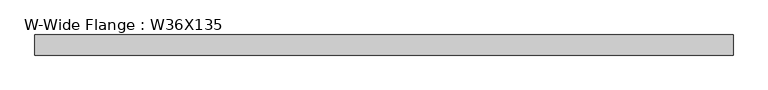
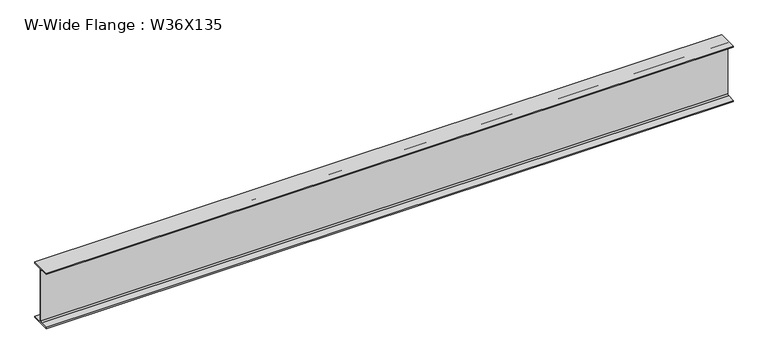
"""IFC4 building model written with IfcOpenShell, lengths in millimetres: beam geometry, W-Wide Flange : W36X135."""

import ifcopenshell
import ifcopenshell.guid

model = None  # the IFC model being written
_history = None  # IfcOwnerHistory: only IFC2X3 demands one
_inside = {}  # id of a spatial element -> (the spatial element, [elements in it])
_under = {}  # id of a project, library or spatial element -> (it, [spatial elements below it])
_declared = {}  # id of a project -> (the project, [libraries it declares])
_typed = {}  # id of a type object -> (the type object, [elements of that type])
_made_of = {}  # id of a material, layer set ... -> (it, [elements and type objects made of it])


def new_model(schema):
    """Start an empty IFC model of exactly this schema.

    Asked for "IFC4X3", IfcOpenShell would pick the latest addendum, in which some entities
    have other attributes; the version numbers below select the first issue.
    IFC2X3 requires an IfcOwnerHistory on every rooted entity: one is made here for all.
    """
    global model, _history
    if schema == "IFC4X3":
        model = ifcopenshell.file(schema_version=(4, 3, 0, 0))
    else:
        model = ifcopenshell.file(schema=schema)
    _inside.clear()
    _under.clear()
    _declared.clear()
    _typed.clear()
    _made_of.clear()
    _history = None
    if model.schema == "IFC2X3":
        org = make("IfcOrganization", Name="unknown")
        user = make(
            "IfcPersonAndOrganization",
            ThePerson=make("IfcPerson", FamilyName="unknown"),
            TheOrganization=org,
        )
        app = make(
            "IfcApplication",
            ApplicationDeveloper=org,
            Version="unknown",
            ApplicationFullName="unknown",
            ApplicationIdentifier="unknown",
        )
        _history = make(
            "IfcOwnerHistory",
            OwningUser=user,
            OwningApplication=app,
            ChangeAction="ADDED",
            CreationDate=0,
        )
    return model


def make(cls, **values):
    """One entity of the class cls with the attributes given. An attribute that is None is left unset."""
    return model.create_entity(
        cls, **{name: value for name, value in values.items() if value is not None}
    )


def rooted(cls, **values):
    """An entity with a GlobalId (a new one), such as an element, a storey or a relation."""
    return make(cls, GlobalId=ifcopenshell.guid.new(), OwnerHistory=_history, **values)


def si_unit(unit_type, name, prefix=None):
    """IfcSIUnit, for example si_unit("LENGTHUNIT", "METRE", prefix="MILLI")."""
    return make("IfcSIUnit", UnitType=unit_type, Prefix=prefix, Name=name)


def assignment(units):
    """IfcUnitAssignment: the units of a project."""
    return None if units is None else make("IfcUnitAssignment", Units=units)


def point(xyz):
    """IfcCartesianPoint."""
    return None if xyz is None else make("IfcCartesianPoint", Coordinates=xyz)


def direction(xyz):
    """IfcDirection."""
    return None if xyz is None else make("IfcDirection", DirectionRatios=xyz)


def frame(location, z_axis=None, x_axis=None):
    """IfcAxis2Placement3D, a coordinate frame: its origin and axes. An axis left out is left unset."""
    return make(
        "IfcAxis2Placement3D",
        Location=point(location),
        Axis=direction(z_axis),
        RefDirection=direction(x_axis),
    )


def frame_2d(location, x_axis=None):
    """IfcAxis2Placement2D, a coordinate frame in the plane: its origin and x axis."""
    return make(
        "IfcAxis2Placement2D", Location=point(location), RefDirection=direction(x_axis)
    )


def origin():
    """The frame at (0, 0, 0) with its axes left unset."""
    return frame((0.0, 0.0, 0.0))


def place(relative_to, where):
    """IfcLocalPlacement: puts the frame where relative to a parent placement (None: the world)."""
    return make(
        "IfcLocalPlacement", PlacementRelTo=relative_to, RelativePlacement=where
    )


def context(
    kind, dimensions, precision=None, world=None, true_north=None, identifier=None
):
    """IfcGeometricRepresentationContext, for example the 3D "Model" context."""
    return make(
        "IfcGeometricRepresentationContext",
        ContextIdentifier=identifier,
        ContextType=kind,
        CoordinateSpaceDimension=dimensions,
        Precision=precision,
        WorldCoordinateSystem=world,
        TrueNorth=true_north,
    )


def project(units=None, contexts=None):
    """IfcProject with its units and contexts."""
    return rooted(
        "IfcProject",
        Name="project",
        RepresentationContexts=contexts,
        UnitsInContext=assignment(units),
    )


def spatial(cls, under=None, at=None, **own):
    """A site, building, storey or space (cls), placed at a placement, below another one or the project."""
    s = rooted(cls, ObjectPlacement=at, **own)
    if under is not None:
        _under.setdefault(under.id(), (under, []))[1].append(s)
    return s


def polyline(points):
    """IfcPolyline through the points."""
    return make("IfcPolyline", Points=[point(p) for p in points])


def circle_curve(where, radius):
    """IfcCircle in the frame where."""
    return make("IfcCircle", Position=where, Radius=radius)


def trimmed(basis, trim1, trim2, sense, master):
    """IfcTrimmedCurve: the piece of a basis curve between two trims."""
    return make(
        "IfcTrimmedCurve",
        BasisCurve=basis,
        Trim1=trim1,
        Trim2=trim2,
        SenseAgreement=sense,
        MasterRepresentation=master,
    )


def segment(curve, same_sense, transition):
    """IfcCompositeCurveSegment."""
    return make(
        "IfcCompositeCurveSegment",
        Transition=transition,
        SameSense=same_sense,
        ParentCurve=curve,
    )


def composite_curve(segments, self_intersect=None):
    """IfcCompositeCurve: segments joined end to end."""
    return make("IfcCompositeCurve", Segments=segments, SelfIntersect=self_intersect)


def outline(outer, holes=None, kind="AREA"):
    """IfcArbitraryClosedProfileDef: a profile drawn as a closed curve; with holes, ...WithVoids."""
    if holes is None:
        return make("IfcArbitraryClosedProfileDef", ProfileType=kind, OuterCurve=outer)
    return make(
        "IfcArbitraryProfileDefWithVoids",
        ProfileType=kind,
        OuterCurve=outer,
        InnerCurves=holes,
    )


def extrude(swept, where, along, depth):
    """IfcExtrudedAreaSolid: the profile swept, set in the frame where, extruded along a direction by depth."""
    return make(
        "IfcExtrudedAreaSolid",
        SweptArea=swept,
        Position=where,
        ExtrudedDirection=direction(along),
        Depth=depth,
    )


def shape(context_of_items, identifier, shape_type, items):
    """IfcShapeRepresentation: the items that make up one representation, for example the "Body"."""
    return make(
        "IfcShapeRepresentation",
        ContextOfItems=context_of_items,
        RepresentationIdentifier=identifier,
        RepresentationType=shape_type,
        Items=items,
    )


def source(mapping_origin, context_of_items, identifier, shape_type, items):
    """IfcRepresentationMap: a shape defined once, which mapped items show again and again."""
    return make(
        "IfcRepresentationMap",
        MappingOrigin=mapping_origin,
        MappedRepresentation=shape(context_of_items, identifier, shape_type, items),
    )


def transform(
    local_origin,
    x_axis=None,
    y_axis=None,
    z_axis=None,
    scale=None,
    scale2=None,
    scale3=None,
    uniform=True,
):
    """IfcCartesianTransformationOperator3D, or its non-uniform kind. x_axis, y_axis, z_axis: its Axis1, 2, 3."""
    if uniform:
        return make(
            "IfcCartesianTransformationOperator3D",
            Axis1=direction(x_axis),
            Axis2=direction(y_axis),
            LocalOrigin=point(local_origin),
            Scale=scale,
            Axis3=direction(z_axis),
        )
    return make(
        "IfcCartesianTransformationOperator3DnonUniform",
        Axis1=direction(x_axis),
        Axis2=direction(y_axis),
        LocalOrigin=point(local_origin),
        Scale=scale,
        Axis3=direction(z_axis),
        Scale2=scale2,
        Scale3=scale3,
    )


def mapped(mapping_source, mapping_target):
    """IfcMappedItem: shows the shape of a source again, moved by a transform."""
    return make(
        "IfcMappedItem", MappingSource=mapping_source, MappingTarget=mapping_target
    )


def made_of(thing, what):
    """Note that an element or type object is made of a material, layer set ...; save() writes the relation."""
    if what is not None:
        _made_of.setdefault(what.id(), (what, []))[1].append(thing)
    return thing


def element(
    cls,
    number,
    at=None,
    inside=None,
    cuts=None,
    type_object=None,
    material=None,
    context=None,
    identifier="Body",
    shape_type=None,
    held_by="IfcProductDefinitionShape",
    body=None,
    shapes=None,
    **own,
):
    """One element of the class cls, such as IfcWall. Its Tag is "e" and its number.

    at: its placement. inside: the storey or other place that contains it. cuts: it is an
    opening in that element (IfcRelVoidsElement). A single representation is given by context,
    identifier, shape_type and body (its items); several are given by shapes. held_by: the class
    of the entity that holds the representations. save() writes the other relations.
    """
    e = rooted(cls, Tag="e%d" % number, ObjectPlacement=at, **own)
    if body is not None:
        shapes = [shape(context, identifier, shape_type, body)]
    if shapes is not None:
        e.Representation = make(held_by, Representations=shapes)
    if inside is not None:
        _inside.setdefault(inside.id(), (inside, []))[1].append(e)
    if cuts is not None:
        rooted(
            "IfcRelVoidsElement", RelatingBuildingElement=cuts, RelatedOpeningElement=e
        )
    if type_object is not None:
        _typed.setdefault(type_object.id(), (type_object, []))[1].append(e)
    return made_of(e, material)


def aggregate(whole, parts):
    """IfcRelAggregates: a whole, such as a stair, and the parts it consists of."""
    return rooted("IfcRelAggregates", RelatingObject=whole, RelatedObjects=parts)


def save(model, path):
    """Write the relations noted so far, then the file.

    IfcRelAggregates (storeys below a building ...), IfcRelContainedInSpatialStructure (elements
    in a storey), IfcRelDefinesByType, IfcRelAssociatesMaterial and IfcRelDeclares: one each for
    every whole, place, type object, material and project.
    """
    for whole, parts in _under.values():
        aggregate(whole, parts)
    for where, things in _inside.values():
        rooted(
            "IfcRelContainedInSpatialStructure",
            RelatedElements=things,
            RelatingStructure=where,
        )
    for kind, things in _typed.values():
        rooted("IfcRelDefinesByType", RelatedObjects=things, RelatingType=kind)
    for what, things in _made_of.values():
        rooted("IfcRelAssociatesMaterial", RelatedObjects=things, RelatingMaterial=what)
    for by, libraries in _declared.values():
        rooted("IfcRelDeclares", RelatingContext=by, RelatedDefinitions=libraries)
    model.write(path)


def w_wide_flange_w36x135_5b543eee(model_context):
    return source(origin(), model_context, "Body", "SweptSolid", [
        extrude(outline(composite_curve([segment(polyline([(152.4, -432.054), (152.4, -452.12), (-152.4, -452.12), (-152.4, -432.054), (-30.4165, -432.054)]), True, "CONTINUOUS"), segment(trimmed(circle_curve(frame_2d((-30.4165, -409.2575)), 22.7965), [point((-30.4165, -432.054))], [point((-7.62, -409.2575))], True, "CARTESIAN"), True, "CONTINUOUS"), segment(polyline([(-7.62, -409.2575), (-7.62, 409.2575)]), True, "CONTINUOUS"), segment(trimmed(circle_curve(frame_2d((-30.4165, 409.2575)), 22.7965), [point((-7.62, 409.2575))], [point((-30.4165, 432.054))], True, "CARTESIAN"), True, "CONTINUOUS"), segment(polyline([(-30.4165, 432.054), (-152.4, 432.054), (-152.4, 452.12), (152.4, 452.12), (152.4, 432.054), (30.4165, 432.054)]), True, "CONTINUOUS"), segment(trimmed(circle_curve(frame_2d((30.4165, 409.2575)), 22.7965), [point((30.4165, 432.054))], [point((7.62, 409.2575))], True, "CARTESIAN"), True, "CONTINUOUS"), segment(polyline([(7.62, 409.2575), (7.62, -409.2575)]), True, "CONTINUOUS"), segment(trimmed(circle_curve(frame_2d((30.4165, -409.2575)), 22.7965), [point((7.62, -409.2575))], [point((30.4165, -432.054))], True, "CARTESIAN"), True, "CONTINUOUS"), segment(polyline([(30.4165, -432.054), (152.4, -432.054)]), True, "CONTINUOUS")], self_intersect=False)), frame((-5347.5061528, 0.0, 0.0), z_axis=(1.0, 0.0, 0.0), x_axis=(0.0, 1.0, 0.0)), (0.0, 0.0, 1.0), 10580.7095618),
    ])


if __name__ == "__main__":
    model = new_model("IFC4")
    model_context = context("Model", 3, world=origin())
    ifc_project = project(units=[si_unit("LENGTHUNIT", "METRE", prefix="MILLI")], contexts=[model_context])
    site = spatial("IfcSite", under=ifc_project)
    building = spatial("IfcBuilding", under=site)
    placement = place(None, origin())
    w_wide_flange_w36x135_shape = w_wide_flange_w36x135_5b543eee(model_context)
    element("IfcBeam", 1, ObjectType="W-Wide Flange : W36X135", at=placement, inside=building, context=model_context, shape_type="MappedRepresentation", body=[
        mapped(w_wide_flange_w36x135_shape, transform((0.0, 0.0, 0.0), x_axis=(1.0, 0.0, 0.0), y_axis=(0.0, 1.0, 0.0), z_axis=(0.0, 0.0, 1.0))),
    ])
    save(model, "model.ifc")

# Revit data of these elements
# Type "W-Wide Flange : W36X135"
#   Assembly Code = "B10"
#   W = 135
#   Length [instance default] = 1524 mm
#   bf = 304.8 mm
#   d = 904.24 mm
#   k = 42.863 mm
#   k2 = 22.797 mm
#   tf = 20.066 mm
#   tw = 15.24 mm
#   A = 0.0256129 m²
#   Structural Material [instance default] = Steel ASTM A992
# Element 1 (IfcBeam, "W-Wide Flange : W36X135")
#   Structural Material = Aluminum, Anodized Red
#   Materials on its faces: "Aluminum, Anodized Red"
# Materials
#   "Steel ASTM A992": class "Metal", colour RGB 128 0 0, transparency 0, Description = "Structural steel 50ksi", Cost = 0
#   "Aluminum, Anodized Red": class "Metal", colour RGB 120 120 120, transparency 0, Description = "Anodized aluminum, red", Cost = 0
